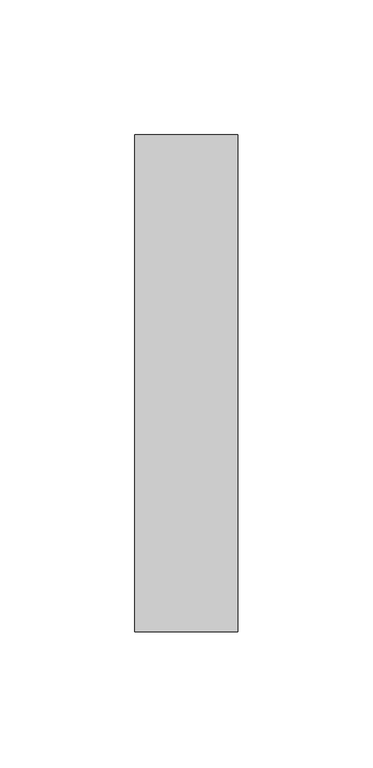
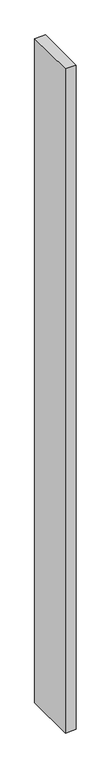
"""IFC4 building model written with IfcOpenShell, lengths in millimetres: proxy geometry, Generic Models 7:Generic Models 1:337419:Generic Models 1:337419 : Generic Models 7:Generic Models 1:337419:51 : Generic Models 7:Generic Models 1:337419:Generic Models 1:337419 : Generic Models 7:Generic Models 1:337419:301336."""

import ifcopenshell
import ifcopenshell.guid

model = None  # the IFC model being written
_history = None  # IfcOwnerHistory: only IFC2X3 demands one
_inside = {}  # id of a spatial element -> (the spatial element, [elements in it])
_under = {}  # id of a project, library or spatial element -> (it, [spatial elements below it])
_declared = {}  # id of a project -> (the project, [libraries it declares])
_typed = {}  # id of a type object -> (the type object, [elements of that type])
_made_of = {}  # id of a material, layer set ... -> (it, [elements and type objects made of it])


def new_model(schema):
    """Start an empty IFC model of exactly this schema.

    Asked for "IFC4X3", IfcOpenShell would pick the latest addendum, in which some entities
    have other attributes; the version numbers below select the first issue.
    IFC2X3 requires an IfcOwnerHistory on every rooted entity: one is made here for all.
    """
    global model, _history
    if schema == "IFC4X3":
        model = ifcopenshell.file(schema_version=(4, 3, 0, 0))
    else:
        model = ifcopenshell.file(schema=schema)
    _inside.clear()
    _under.clear()
    _declared.clear()
    _typed.clear()
    _made_of.clear()
    _history = None
    if model.schema == "IFC2X3":
        org = make("IfcOrganization", Name="unknown")
        user = make(
            "IfcPersonAndOrganization",
            ThePerson=make("IfcPerson", FamilyName="unknown"),
            TheOrganization=org,
        )
        app = make(
            "IfcApplication",
            ApplicationDeveloper=org,
            Version="unknown",
            ApplicationFullName="unknown",
            ApplicationIdentifier="unknown",
        )
        _history = make(
            "IfcOwnerHistory",
            OwningUser=user,
            OwningApplication=app,
            ChangeAction="ADDED",
            CreationDate=0,
        )
    return model


def make(cls, **values):
    """One entity of the class cls with the attributes given. An attribute that is None is left unset."""
    return model.create_entity(
        cls, **{name: value for name, value in values.items() if value is not None}
    )


def rooted(cls, **values):
    """An entity with a GlobalId (a new one), such as an element, a storey or a relation."""
    return make(cls, GlobalId=ifcopenshell.guid.new(), OwnerHistory=_history, **values)


def si_unit(unit_type, name, prefix=None):
    """IfcSIUnit, for example si_unit("LENGTHUNIT", "METRE", prefix="MILLI")."""
    return make("IfcSIUnit", UnitType=unit_type, Prefix=prefix, Name=name)


def assignment(units):
    """IfcUnitAssignment: the units of a project."""
    return None if units is None else make("IfcUnitAssignment", Units=units)


def point(xyz):
    """IfcCartesianPoint."""
    return None if xyz is None else make("IfcCartesianPoint", Coordinates=xyz)


def direction(xyz):
    """IfcDirection."""
    return None if xyz is None else make("IfcDirection", DirectionRatios=xyz)


def frame(location, z_axis=None, x_axis=None):
    """IfcAxis2Placement3D, a coordinate frame: its origin and axes. An axis left out is left unset."""
    return make(
        "IfcAxis2Placement3D",
        Location=point(location),
        Axis=direction(z_axis),
        RefDirection=direction(x_axis),
    )


def origin():
    """The frame at (0, 0, 0) with its axes left unset."""
    return frame((0.0, 0.0, 0.0))


def origin_with_axes():
    """The frame at (0, 0, 0) with the z axis (0, 0, 1) and the x axis (1, 0, 0) written out."""
    return frame((0.0, 0.0, 0.0), z_axis=(0.0, 0.0, 1.0), x_axis=(1.0, 0.0, 0.0))


def place(relative_to, where):
    """IfcLocalPlacement: puts the frame where relative to a parent placement (None: the world)."""
    return make(
        "IfcLocalPlacement", PlacementRelTo=relative_to, RelativePlacement=where
    )


def context(
    kind, dimensions, precision=None, world=None, true_north=None, identifier=None
):
    """IfcGeometricRepresentationContext, for example the 3D "Model" context."""
    return make(
        "IfcGeometricRepresentationContext",
        ContextIdentifier=identifier,
        ContextType=kind,
        CoordinateSpaceDimension=dimensions,
        Precision=precision,
        WorldCoordinateSystem=world,
        TrueNorth=true_north,
    )


def project(units=None, contexts=None):
    """IfcProject with its units and contexts."""
    return rooted(
        "IfcProject",
        Name="project",
        RepresentationContexts=contexts,
        UnitsInContext=assignment(units),
    )


def spatial(cls, under=None, at=None, **own):
    """A site, building, storey or space (cls), placed at a placement, below another one or the project."""
    s = rooted(cls, ObjectPlacement=at, **own)
    if under is not None:
        _under.setdefault(under.id(), (under, []))[1].append(s)
    return s


def polyline(points):
    """IfcPolyline through the points."""
    return make("IfcPolyline", Points=[point(p) for p in points])


def outline(outer, holes=None, kind="AREA"):
    """IfcArbitraryClosedProfileDef: a profile drawn as a closed curve; with holes, ...WithVoids."""
    if holes is None:
        return make("IfcArbitraryClosedProfileDef", ProfileType=kind, OuterCurve=outer)
    return make(
        "IfcArbitraryProfileDefWithVoids",
        ProfileType=kind,
        OuterCurve=outer,
        InnerCurves=holes,
    )


def extrude(swept, where, along, depth):
    """IfcExtrudedAreaSolid: the profile swept, set in the frame where, extruded along a direction by depth."""
    return make(
        "IfcExtrudedAreaSolid",
        SweptArea=swept,
        Position=where,
        ExtrudedDirection=direction(along),
        Depth=depth,
    )


def shape(context_of_items, identifier, shape_type, items):
    """IfcShapeRepresentation: the items that make up one representation, for example the "Body"."""
    return make(
        "IfcShapeRepresentation",
        ContextOfItems=context_of_items,
        RepresentationIdentifier=identifier,
        RepresentationType=shape_type,
        Items=items,
    )


def source(mapping_origin, context_of_items, identifier, shape_type, items):
    """IfcRepresentationMap: a shape defined once, which mapped items show again and again."""
    return make(
        "IfcRepresentationMap",
        MappingOrigin=mapping_origin,
        MappedRepresentation=shape(context_of_items, identifier, shape_type, items),
    )


def transform(
    local_origin,
    x_axis=None,
    y_axis=None,
    z_axis=None,
    scale=None,
    scale2=None,
    scale3=None,
    uniform=True,
):
    """IfcCartesianTransformationOperator3D, or its non-uniform kind. x_axis, y_axis, z_axis: its Axis1, 2, 3."""
    if uniform:
        return make(
            "IfcCartesianTransformationOperator3D",
            Axis1=direction(x_axis),
            Axis2=direction(y_axis),
            LocalOrigin=point(local_origin),
            Scale=scale,
            Axis3=direction(z_axis),
        )
    return make(
        "IfcCartesianTransformationOperator3DnonUniform",
        Axis1=direction(x_axis),
        Axis2=direction(y_axis),
        LocalOrigin=point(local_origin),
        Scale=scale,
        Axis3=direction(z_axis),
        Scale2=scale2,
        Scale3=scale3,
    )


def mapped(mapping_source, mapping_target):
    """IfcMappedItem: shows the shape of a source again, moved by a transform."""
    return make(
        "IfcMappedItem", MappingSource=mapping_source, MappingTarget=mapping_target
    )


def made_of(thing, what):
    """Note that an element or type object is made of a material, layer set ...; save() writes the relation."""
    if what is not None:
        _made_of.setdefault(what.id(), (what, []))[1].append(thing)
    return thing


def element(
    cls,
    number,
    at=None,
    inside=None,
    cuts=None,
    type_object=None,
    material=None,
    context=None,
    identifier="Body",
    shape_type=None,
    held_by="IfcProductDefinitionShape",
    body=None,
    shapes=None,
    **own,
):
    """One element of the class cls, such as IfcWall. Its Tag is "e" and its number.

    at: its placement. inside: the storey or other place that contains it. cuts: it is an
    opening in that element (IfcRelVoidsElement). A single representation is given by context,
    identifier, shape_type and body (its items); several are given by shapes. held_by: the class
    of the entity that holds the representations. save() writes the other relations.
    """
    e = rooted(cls, Tag="e%d" % number, ObjectPlacement=at, **own)
    if body is not None:
        shapes = [shape(context, identifier, shape_type, body)]
    if shapes is not None:
        e.Representation = make(held_by, Representations=shapes)
    if inside is not None:
        _inside.setdefault(inside.id(), (inside, []))[1].append(e)
    if cuts is not None:
        rooted(
            "IfcRelVoidsElement", RelatingBuildingElement=cuts, RelatedOpeningElement=e
        )
    if type_object is not None:
        _typed.setdefault(type_object.id(), (type_object, []))[1].append(e)
    return made_of(e, material)


def aggregate(whole, parts):
    """IfcRelAggregates: a whole, such as a stair, and the parts it consists of."""
    return rooted("IfcRelAggregates", RelatingObject=whole, RelatedObjects=parts)


def save(model, path):
    """Write the relations noted so far, then the file.

    IfcRelAggregates (storeys below a building ...), IfcRelContainedInSpatialStructure (elements
    in a storey), IfcRelDefinesByType, IfcRelAssociatesMaterial and IfcRelDeclares: one each for
    every whole, place, type object, material and project.
    """
    for whole, parts in _under.values():
        aggregate(whole, parts)
    for where, things in _inside.values():
        rooted(
            "IfcRelContainedInSpatialStructure",
            RelatedElements=things,
            RelatingStructure=where,
        )
    for kind, things in _typed.values():
        rooted("IfcRelDefinesByType", RelatedObjects=things, RelatingType=kind)
    for what, things in _made_of.values():
        rooted("IfcRelAssociatesMaterial", RelatedObjects=things, RelatingMaterial=what)
    for by, libraries in _declared.values():
        rooted("IfcRelDeclares", RelatingContext=by, RelatedDefinitions=libraries)
    model.write(path)


def generic_models_b4d7931b(model_context):
    return source(origin(), model_context, "Body", "SweptSolid", [
        extrude(outline(polyline([(593892.203627, -536785.4956512), (593854.103627, -536785.4956512), (593854.103627, -536601.3456512), (593892.203627, -536601.3456512), (593892.203627, -536785.4956512)])), origin_with_axes(), (0.0, 0.0, 1.0), 2438.4),
    ])


if __name__ == "__main__":
    model = new_model("IFC4")
    model_context = context("Model", 3, world=origin())
    ifc_project = project(units=[si_unit("LENGTHUNIT", "METRE", prefix="MILLI")], contexts=[model_context])
    site = spatial("IfcSite", under=ifc_project)
    building = spatial("IfcBuilding", under=site)
    placement = place(None, origin())
    generic_models_shape = generic_models_b4d7931b(model_context)
    element("IfcBuildingElementProxy", 1, Name="Generic Models 7:Generic Models 1:337419:Generic Models 1:337419 : Generic Models 7:Generic Models 1:337419:51 : Generic Models 7:Generic Models 1:337419:Generic Models 1:337419 : Generic Models 7:Generic Models 1:337419:301336", ObjectType="Generic Models 7:Generic Models 1:337419:Generic Models 1:337419 : Generic Models 7:Generic Models 1:337419:51 : Generic Models 7:Generic Models 1:337419:Generic Models 1:337419 : Generic Models 7:Generic Models 1:337419:301336", at=placement, inside=building, context=model_context, shape_type="MappedRepresentation", body=[
        mapped(generic_models_shape, transform((0.0, 0.0, 0.0), x_axis=(1.0, 0.0, 0.0), y_axis=(0.0, 1.0, 0.0), z_axis=(0.0, 0.0, 1.0))),
    ])
    save(model, "model.ifc")

# Revit data of these elements
# Type "Generic Models 7:Generic Models 1:337419:Generic Models 1:337419 : Generic Models 7:Generic Models 1:337419:51 : Generic Models 7:Generic Models 1:337419:Generic Models 1:337419 : Generic Models 7:Generic Models 1:337419:301336"
#   NameOverride = "Generic Models 7:Generic Models 1:337419:Generic Models 1:337419 : Generic Models 7:Generic Models 1:337419:301336"
#   ObjectTypeOverride = "Generic Models 1:337419 : Generic Models 7:Generic Models 1:337419"
#   Reference = "Generic Models 1"
#   Tag = "301336"
# Element 1 (IfcBuildingElementProxy, "Generic Models 7:Generic Models 1:337419:Generic Models 1:337419 : Generic Models 7:Generic Models 1:337419:51 : Generic Models 7:Generic Models 1:337419:Generic Models 1:337419 : Generic Models 7:Generic Models 1:337419:301336")
#   Materials on its faces: "BLOCKING - SIZE AS NEC."
# Materials
#   "BLOCKING - SIZE AS NEC.": class "Wood", colour RGB 144 113 62, transparency 0, Description = "Pinus Echinata", Cost = 0
